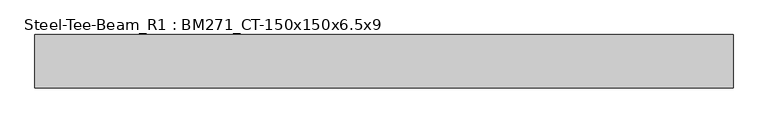
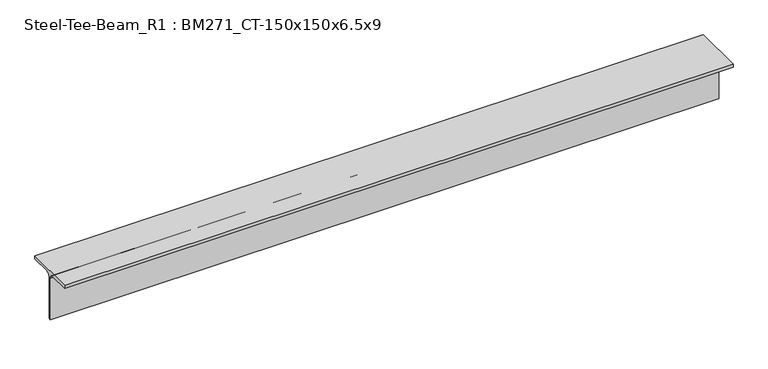
"""IFC4 building model written with IfcOpenShell, lengths in millimetres: member geometry, Steel-Tee-Beam_R1 : BM271_CT-150x150x6.5x9."""

from ifc_helpers import new_model, si_unit, point, frame, frame_2d, origin, place, context, project, spatial, polyline, circle_curve, trimmed, segment, composite_curve, outline, extrude, source, transform, mapped, element, save


def steel_tee_beam_r1_bm271_ct_150x150x6_5x9_a9d363ab(model_context):
    return source(origin(), model_context, "Body", "SweptSolid", [
        extrude(outline(composite_curve([segment(polyline([(75.0, 75.0), (75.0, 66.0), (16.25, 66.0)]), True, "CONTINUOUS"), segment(trimmed(circle_curve(frame_2d((16.25, 53.0)), 13.0), [point((16.25, 66.0))], [point((3.25, 53.0))], True, "CARTESIAN"), True, "CONTINUOUS"), segment(polyline([(3.25, 53.0), (3.25, -75.0), (-3.25, -75.0), (-3.25, 53.0)]), True, "CONTINUOUS"), segment(trimmed(circle_curve(frame_2d((-16.25, 53.0)), 13.0), [point((-3.25, 53.0))], [point((-16.25, 66.0))], True, "CARTESIAN"), True, "CONTINUOUS"), segment(polyline([(-16.25, 66.0), (-75.0, 66.0), (-75.0, 75.0), (75.0, 75.0)]), True, "CONTINUOUS")], self_intersect=False)), frame((-1113.6541462, 0.0, 0.0), z_axis=(1.0, 0.0, 0.0), x_axis=(0.0, 1.0, 0.0)), (0.0, 0.0, 1.0), 1955.9770441),
    ])


if __name__ == "__main__":
    model = new_model("IFC4")
    model_context = context("Model", 3, world=origin())
    ifc_project = project(units=[si_unit("LENGTHUNIT", "METRE", prefix="MILLI")], contexts=[model_context])
    site = spatial("IfcSite", under=ifc_project)
    building = spatial("IfcBuilding", under=site)
    placement = place(None, origin())
    steel_tee_beam_r1_bm271_ct_150x150x6_5x9_shape = steel_tee_beam_r1_bm271_ct_150x150x6_5x9_a9d363ab(model_context)
    element("IfcMember", 1, ObjectType="Steel-Tee-Beam_R1 : BM271_CT-150x150x6.5x9", at=placement, inside=building, context=model_context, shape_type="MappedRepresentation", body=[
        mapped(steel_tee_beam_r1_bm271_ct_150x150x6_5x9_shape, transform((0.0, 0.0, 0.0), x_axis=(1.0, 0.0, 0.0), y_axis=(0.0, 1.0, 0.0), z_axis=(0.0, 0.0, 1.0))),
    ])
    save(model, "model.ifc")

# Revit data of these elements
# Type "Steel-Tee-Beam_R1 : BM271_CT-150x150x6.5x9"
#   Keynote = "CT-150x150x6.5x9"
#   Surface Area = 0.588841 m²/m
#   Section Area = 23.3904 cm²
#   Mass per Unit Length = 18.3614 kg/m
#   Length [instance default] = 1.5240 m
#   bf = 0.1500 m
#   d = 0.1500 m
#   k = 0.0220 m
#   r = 0.0130 m
#   tf = 0.0090 m
#   tw = 0.0065 m
#   hec_material4 [instance default] = none
#   hec_material3 [instance default] = none
#   hec_material2 [instance default] = none
#   hec_material1 [instance default] = none
#   Structural Material [instance default] = Steel, 45-345
#   Assembly Code = ""
# Element 1 (IfcMember, "Steel-Tee-Beam_R1 : BM271_CT-150x150x6.5x9")
#   Structural Material = none
# Materials
#   "Steel, 45-345": class "Metal", colour RGB 189 187 185, transparency 0, Description = "Steel 345 MPa", Cost = 0
